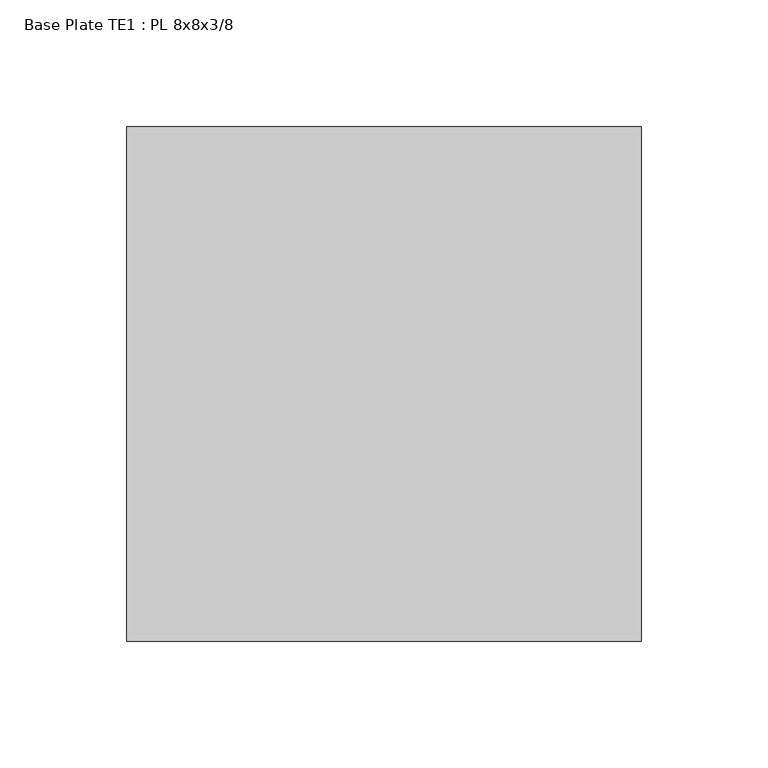
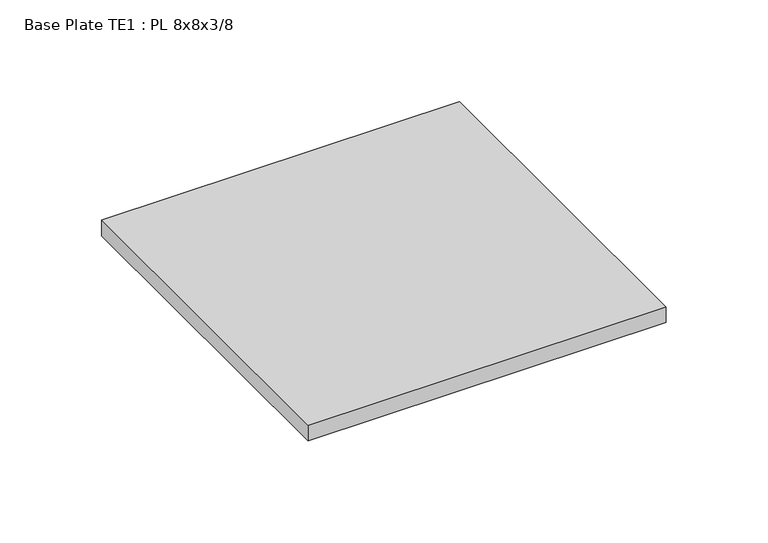
"""IFC4 building model written with IfcOpenShell, lengths in millimetres: proxy geometry, Base Plate TE1 : PL 8x8x3/8."""

import ifcopenshell
import ifcopenshell.guid

model = None  # the IFC model being written
_history = None  # IfcOwnerHistory: only IFC2X3 demands one
_inside = {}  # id of a spatial element -> (the spatial element, [elements in it])
_under = {}  # id of a project, library or spatial element -> (it, [spatial elements below it])
_declared = {}  # id of a project -> (the project, [libraries it declares])
_typed = {}  # id of a type object -> (the type object, [elements of that type])
_made_of = {}  # id of a material, layer set ... -> (it, [elements and type objects made of it])


def new_model(schema):
    """Start an empty IFC model of exactly this schema.

    Asked for "IFC4X3", IfcOpenShell would pick the latest addendum, in which some entities
    have other attributes; the version numbers below select the first issue.
    IFC2X3 requires an IfcOwnerHistory on every rooted entity: one is made here for all.
    """
    global model, _history
    if schema == "IFC4X3":
        model = ifcopenshell.file(schema_version=(4, 3, 0, 0))
    else:
        model = ifcopenshell.file(schema=schema)
    _inside.clear()
    _under.clear()
    _declared.clear()
    _typed.clear()
    _made_of.clear()
    _history = None
    if model.schema == "IFC2X3":
        org = make("IfcOrganization", Name="unknown")
        user = make(
            "IfcPersonAndOrganization",
            ThePerson=make("IfcPerson", FamilyName="unknown"),
            TheOrganization=org,
        )
        app = make(
            "IfcApplication",
            ApplicationDeveloper=org,
            Version="unknown",
            ApplicationFullName="unknown",
            ApplicationIdentifier="unknown",
        )
        _history = make(
            "IfcOwnerHistory",
            OwningUser=user,
            OwningApplication=app,
            ChangeAction="ADDED",
            CreationDate=0,
        )
    return model


def make(cls, **values):
    """One entity of the class cls with the attributes given. An attribute that is None is left unset."""
    return model.create_entity(
        cls, **{name: value for name, value in values.items() if value is not None}
    )


def rooted(cls, **values):
    """An entity with a GlobalId (a new one), such as an element, a storey or a relation."""
    return make(cls, GlobalId=ifcopenshell.guid.new(), OwnerHistory=_history, **values)


def si_unit(unit_type, name, prefix=None):
    """IfcSIUnit, for example si_unit("LENGTHUNIT", "METRE", prefix="MILLI")."""
    return make("IfcSIUnit", UnitType=unit_type, Prefix=prefix, Name=name)


def assignment(units):
    """IfcUnitAssignment: the units of a project."""
    return None if units is None else make("IfcUnitAssignment", Units=units)


def point(xyz):
    """IfcCartesianPoint."""
    return None if xyz is None else make("IfcCartesianPoint", Coordinates=xyz)


def direction(xyz):
    """IfcDirection."""
    return None if xyz is None else make("IfcDirection", DirectionRatios=xyz)


def frame(location, z_axis=None, x_axis=None):
    """IfcAxis2Placement3D, a coordinate frame: its origin and axes. An axis left out is left unset."""
    return make(
        "IfcAxis2Placement3D",
        Location=point(location),
        Axis=direction(z_axis),
        RefDirection=direction(x_axis),
    )


def origin():
    """The frame at (0, 0, 0) with its axes left unset."""
    return frame((0.0, 0.0, 0.0))


def place(relative_to, where):
    """IfcLocalPlacement: puts the frame where relative to a parent placement (None: the world)."""
    return make(
        "IfcLocalPlacement", PlacementRelTo=relative_to, RelativePlacement=where
    )


def context(
    kind, dimensions, precision=None, world=None, true_north=None, identifier=None
):
    """IfcGeometricRepresentationContext, for example the 3D "Model" context."""
    return make(
        "IfcGeometricRepresentationContext",
        ContextIdentifier=identifier,
        ContextType=kind,
        CoordinateSpaceDimension=dimensions,
        Precision=precision,
        WorldCoordinateSystem=world,
        TrueNorth=true_north,
    )


def project(units=None, contexts=None):
    """IfcProject with its units and contexts."""
    return rooted(
        "IfcProject",
        Name="project",
        RepresentationContexts=contexts,
        UnitsInContext=assignment(units),
    )


def spatial(cls, under=None, at=None, **own):
    """A site, building, storey or space (cls), placed at a placement, below another one or the project."""
    s = rooted(cls, ObjectPlacement=at, **own)
    if under is not None:
        _under.setdefault(under.id(), (under, []))[1].append(s)
    return s


def polyline(points):
    """IfcPolyline through the points."""
    return make("IfcPolyline", Points=[point(p) for p in points])


def outline(outer, holes=None, kind="AREA"):
    """IfcArbitraryClosedProfileDef: a profile drawn as a closed curve; with holes, ...WithVoids."""
    if holes is None:
        return make("IfcArbitraryClosedProfileDef", ProfileType=kind, OuterCurve=outer)
    return make(
        "IfcArbitraryProfileDefWithVoids",
        ProfileType=kind,
        OuterCurve=outer,
        InnerCurves=holes,
    )


def extrude(swept, where, along, depth):
    """IfcExtrudedAreaSolid: the profile swept, set in the frame where, extruded along a direction by depth."""
    return make(
        "IfcExtrudedAreaSolid",
        SweptArea=swept,
        Position=where,
        ExtrudedDirection=direction(along),
        Depth=depth,
    )


def shape(context_of_items, identifier, shape_type, items):
    """IfcShapeRepresentation: the items that make up one representation, for example the "Body"."""
    return make(
        "IfcShapeRepresentation",
        ContextOfItems=context_of_items,
        RepresentationIdentifier=identifier,
        RepresentationType=shape_type,
        Items=items,
    )


def source(mapping_origin, context_of_items, identifier, shape_type, items):
    """IfcRepresentationMap: a shape defined once, which mapped items show again and again."""
    return make(
        "IfcRepresentationMap",
        MappingOrigin=mapping_origin,
        MappedRepresentation=shape(context_of_items, identifier, shape_type, items),
    )


def transform(
    local_origin,
    x_axis=None,
    y_axis=None,
    z_axis=None,
    scale=None,
    scale2=None,
    scale3=None,
    uniform=True,
):
    """IfcCartesianTransformationOperator3D, or its non-uniform kind. x_axis, y_axis, z_axis: its Axis1, 2, 3."""
    if uniform:
        return make(
            "IfcCartesianTransformationOperator3D",
            Axis1=direction(x_axis),
            Axis2=direction(y_axis),
            LocalOrigin=point(local_origin),
            Scale=scale,
            Axis3=direction(z_axis),
        )
    return make(
        "IfcCartesianTransformationOperator3DnonUniform",
        Axis1=direction(x_axis),
        Axis2=direction(y_axis),
        LocalOrigin=point(local_origin),
        Scale=scale,
        Axis3=direction(z_axis),
        Scale2=scale2,
        Scale3=scale3,
    )


def mapped(mapping_source, mapping_target):
    """IfcMappedItem: shows the shape of a source again, moved by a transform."""
    return make(
        "IfcMappedItem", MappingSource=mapping_source, MappingTarget=mapping_target
    )


def made_of(thing, what):
    """Note that an element or type object is made of a material, layer set ...; save() writes the relation."""
    if what is not None:
        _made_of.setdefault(what.id(), (what, []))[1].append(thing)
    return thing


def element(
    cls,
    number,
    at=None,
    inside=None,
    cuts=None,
    type_object=None,
    material=None,
    context=None,
    identifier="Body",
    shape_type=None,
    held_by="IfcProductDefinitionShape",
    body=None,
    shapes=None,
    **own,
):
    """One element of the class cls, such as IfcWall. Its Tag is "e" and its number.

    at: its placement. inside: the storey or other place that contains it. cuts: it is an
    opening in that element (IfcRelVoidsElement). A single representation is given by context,
    identifier, shape_type and body (its items); several are given by shapes. held_by: the class
    of the entity that holds the representations. save() writes the other relations.
    """
    e = rooted(cls, Tag="e%d" % number, ObjectPlacement=at, **own)
    if body is not None:
        shapes = [shape(context, identifier, shape_type, body)]
    if shapes is not None:
        e.Representation = make(held_by, Representations=shapes)
    if inside is not None:
        _inside.setdefault(inside.id(), (inside, []))[1].append(e)
    if cuts is not None:
        rooted(
            "IfcRelVoidsElement", RelatingBuildingElement=cuts, RelatedOpeningElement=e
        )
    if type_object is not None:
        _typed.setdefault(type_object.id(), (type_object, []))[1].append(e)
    return made_of(e, material)


def aggregate(whole, parts):
    """IfcRelAggregates: a whole, such as a stair, and the parts it consists of."""
    return rooted("IfcRelAggregates", RelatingObject=whole, RelatedObjects=parts)


def save(model, path):
    """Write the relations noted so far, then the file.

    IfcRelAggregates (storeys below a building ...), IfcRelContainedInSpatialStructure (elements
    in a storey), IfcRelDefinesByType, IfcRelAssociatesMaterial and IfcRelDeclares: one each for
    every whole, place, type object, material and project.
    """
    for whole, parts in _under.values():
        aggregate(whole, parts)
    for where, things in _inside.values():
        rooted(
            "IfcRelContainedInSpatialStructure",
            RelatedElements=things,
            RelatingStructure=where,
        )
    for kind, things in _typed.values():
        rooted("IfcRelDefinesByType", RelatedObjects=things, RelatingType=kind)
    for what, things in _made_of.values():
        rooted("IfcRelAssociatesMaterial", RelatedObjects=things, RelatingMaterial=what)
    for by, libraries in _declared.values():
        rooted("IfcRelDeclares", RelatingContext=by, RelatedDefinitions=libraries)
    model.write(path)


def base_plate_te1_pl_8x8x3_8_a06680a7(model_context):
    return source(origin(), model_context, "Body", "SweptSolid", [
        extrude(outline(polyline([(590318.6599233, -532779.0413841), (590318.6599233, -532982.2413841), (590115.4599233, -532982.2413841), (590115.4599233, -532779.0413841), (590318.6599233, -532779.0413841)])), frame((0.0, 0.0, 19.05), z_axis=(0.0, 0.0, 1.0), x_axis=(1.0, 0.0, 0.0)), (0.0, 0.0, 1.0), 9.525),
    ])


if __name__ == "__main__":
    model = new_model("IFC4")
    model_context = context("Model", 3, world=origin())
    ifc_project = project(units=[si_unit("LENGTHUNIT", "METRE", prefix="MILLI")], contexts=[model_context])
    site = spatial("IfcSite", under=ifc_project)
    building = spatial("IfcBuilding", under=site)
    placement = place(None, origin())
    base_plate_te1_pl_8x8x3_8_shape = base_plate_te1_pl_8x8x3_8_a06680a7(model_context)
    element("IfcBuildingElementProxy", 1, Name="Base Plate TE1 : PL 8x8x3/8", ObjectType="Base Plate TE1 : PL 8x8x3/8", at=placement, inside=building, context=model_context, shape_type="MappedRepresentation", body=[
        mapped(base_plate_te1_pl_8x8x3_8_shape, transform((0.0, 0.0, 0.0), x_axis=(1.0, 0.0, 0.0), y_axis=(0.0, 1.0, 0.0), z_axis=(0.0, 0.0, 1.0))),
    ])
    save(model, "model.ifc")

# Revit data of these elements
# Element 1 (IfcBuildingElementProxy, "Base Plate TE1 : PL 8x8x3/8")
#   Materials on its faces: "GALV. STL BASE PLATE"
# Materials
#   "GALV. STL BASE PLATE": class "Generic", colour RGB 211 211 207, transparency 0, Cost = 0
